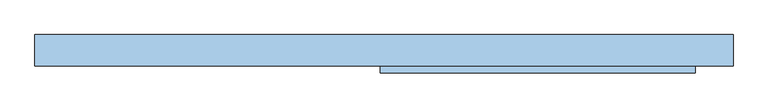
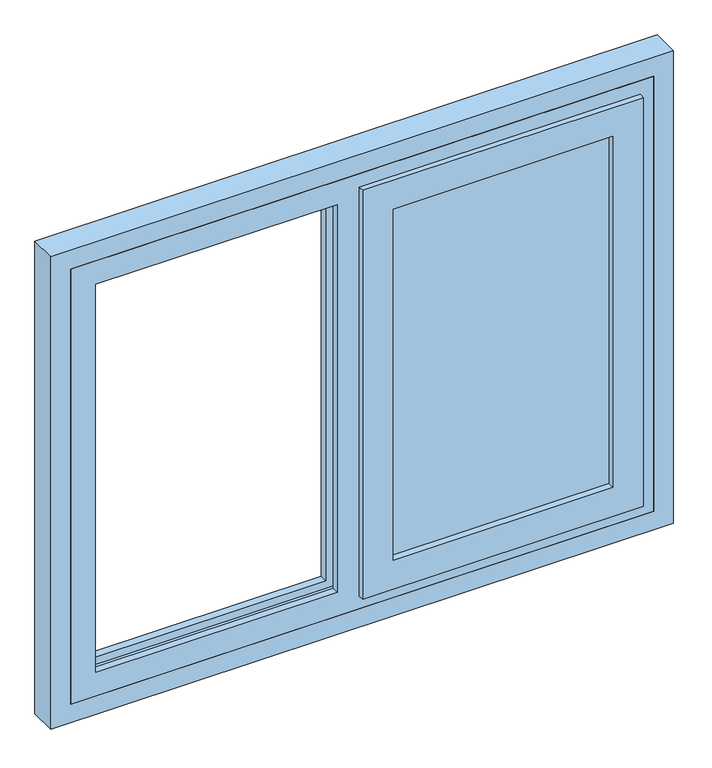
"""IFC4 building model written with IfcOpenShell, lengths in millimetres: window geometry, Окно 2-Откидное - Левое глухое - Один переплет с многокамерным стеклопакетом - 30674-99 : ОП Г1  1160-1540 (4M1-10-4M1-10-4M1) ГОСТ 30674-99."""

from ifc_helpers import new_model, si_unit, frame, origin, place, context, project, spatial, polyline, outline, extrude, faceted_brep, source, transform, mapped, element, save


def window_171b5b07(model_context):
    return source(origin(), model_context, "Body", "SolidModel", [
        extrude(outline(polyline([(942.0, 643.0), (1918.0, 643.0), (1918.0, 49.0), (942.0, 49.0), (942.0, 643.0)]), holes=[polyline([(1903.0, 628.0), (957.0, 628.0), (957.0, 64.0), (1903.0, 64.0), (1903.0, 628.0)])]), frame((0.0, 140.0, 0.0), z_axis=(0.0, 1.0, 0.0), x_axis=(0.0, 0.0, 1.0)), (0.0, 0.0, 1.0), 10.0),
        extrude(outline(polyline([(942.0, 643.0), (1918.0, 643.0), (1918.0, 49.0), (942.0, 49.0), (942.0, 643.0)]), holes=[polyline([(1903.0, 628.0), (957.0, 628.0), (957.0, 64.0), (1903.0, 64.0), (1903.0, 628.0)])]), frame((0.0, 126.0, 0.0), z_axis=(0.0, 1.0, 0.0), x_axis=(0.0, 0.0, 1.0)), (0.0, 0.0, 1.0), 10.0),
        extrude(outline(polyline([(49.0, 140.0), (643.0, 140.0), (643.0, 136.0), (49.0, 136.0), (49.0, 140.0)])), frame((0.0, 0.0, 942.0), z_axis=(0.0, 0.0, 1.0), x_axis=(1.0, 0.0, 0.0)), (0.0, 0.0, 1.0), 976.0),
        extrude(outline(polyline([(49.0, 154.0), (643.0, 154.0), (643.0, 150.0), (49.0, 150.0), (49.0, 154.0)])), frame((0.0, 0.0, 942.0), z_axis=(0.0, 0.0, 1.0), x_axis=(1.0, 0.0, 0.0)), (0.0, 0.0, 1.0), 976.0),
        extrude(outline(polyline([(49.0, 126.0), (643.0, 126.0), (643.0, 122.0), (49.0, 122.0), (49.0, 126.0)])), frame((0.0, 0.0, 942.0), z_axis=(0.0, 0.0, 1.0), x_axis=(1.0, 0.0, 0.0)), (0.0, 0.0, 1.0), 976.0),
        faceted_brep([(-735.0, 120.0, 2010.0), (-735.0, 190.0, 2010.0), (-735.0, 190.0, 850.0), (-735.0, 120.0, 850.0), (735.0, 190.0, 850.0), (735.0, 190.0, 2010.0), (-672.0, 190.0, 1947.0), (-672.0, 190.0, 913.0), (-63.0, 190.0, 913.0), (-63.0, 190.0, 1947.0), (19.0, 190.0, 1947.0), (19.0, 190.0, 913.0), (672.0, 190.0, 913.0), (672.0, 190.0, 1947.0), (735.0, 120.0, 850.0), (735.0, 120.0, 2010.0), (-672.0, 120.0, 913.0), (-672.0, 120.0, 1947.0), (-63.0, 120.0, 1947.0), (-63.0, 120.0, 913.0), (0.0, 120.0, 893.0), (0.0, 120.0, 1967.0), (692.0, 120.0, 1967.0), (692.0, 120.0, 893.0), (-672.0, 138.0, 1947.0), (-672.0, 138.0, 913.0), (-63.0, 138.0, 913.0), (-692.0, 138.0, 893.0), (-692.0, 138.0, 1967.0), (-43.0, 138.0, 1967.0), (-43.0, 138.0, 893.0), (-63.0, 138.0, 1947.0), (-692.0, 170.0, 1967.0), (-692.0, 170.0, 893.0), (-43.0, 170.0, 893.0), (-43.0, 170.0, 1967.0), (-672.0, 170.0, 913.0), (-672.0, 170.0, 1947.0), (-63.0, 170.0, 1947.0), (-63.0, 170.0, 913.0), (0.0, 176.0, 893.0), (0.0, 176.0, 1967.0), (692.0, 176.0, 893.0), (692.0, 176.0, 1967.0), (19.0, 176.0, 913.0), (19.0, 176.0, 1947.0), (672.0, 176.0, 1947.0), (672.0, 176.0, 913.0)], [[[0, 1, 2, 3]], [[4, 2, 1, 5], [6, 7, 8, 9], [10, 11, 12, 13]], [[3, 2, 4, 14]], [[15, 0, 3, 14], [16, 17, 18, 19], [20, 21, 22, 23]], [[24, 17, 16, 25]], [[25, 16, 19, 26]], [[27, 28, 29, 30], [24, 25, 26, 31]], [[32, 28, 27, 33]], [[33, 27, 30, 34]], [[32, 33, 34, 35], [36, 37, 38, 39]], [[6, 37, 36, 7]], [[7, 36, 39, 8]], [[15, 14, 4, 5]], [[26, 19, 18, 31]], [[34, 30, 29, 35]], [[8, 39, 38, 9]], [[40, 41, 21, 20]], [[42, 43, 41, 40], [44, 45, 46, 47]], [[20, 23, 42, 40]], [[11, 10, 45, 44]], [[47, 12, 11, 44]], [[46, 13, 12, 47]], [[43, 42, 23, 22]], [[5, 1, 0, 15]], [[17, 24, 31, 18]], [[28, 32, 35, 29]], [[37, 6, 9, 38]], [[13, 46, 45, 10]], [[41, 43, 22, 21]]]),
        faceted_brep([(69.0, 174.0, 1898.0), (69.0, 154.0, 1898.0), (69.0, 154.0, 962.0), (69.0, 174.0, 962.0), (49.0, 154.0, 942.0), (643.0, 154.0, 942.0), (643.0, 154.0, 1918.0), (49.0, 154.0, 1918.0), (623.0, 154.0, 1898.0), (623.0, 154.0, 962.0), (623.0, 174.0, 962.0), (12.0, 174.0, 1955.0), (680.0, 174.0, 1955.0), (680.0, 174.0, 905.0), (12.0, 174.0, 905.0), (623.0, 174.0, 1898.0), (12.0, 118.0, 1955.0), (12.0, 118.0, 905.0), (680.0, 118.0, 905.0), (-8.0, 118.0, 1975.0), (700.0, 118.0, 1975.0), (700.0, 118.0, 885.0), (-8.0, 118.0, 885.0), (680.0, 118.0, 1955.0), (-8.0, 104.0, 1975.0), (-8.0, 104.0, 885.0), (700.0, 104.0, 885.0), (700.0, 104.0, 1975.0), (69.0, 104.0, 1898.0), (623.0, 104.0, 1898.0), (623.0, 104.0, 962.0), (69.0, 104.0, 962.0), (69.0, 122.0, 1898.0), (69.0, 122.0, 962.0), (623.0, 122.0, 962.0), (49.0, 122.0, 1918.0), (643.0, 122.0, 1918.0), (643.0, 122.0, 942.0), (49.0, 122.0, 942.0), (623.0, 122.0, 1898.0)], [[[0, 1, 2, 3]], [[4, 5, 6, 7], [1, 8, 9, 2]], [[3, 2, 9, 10]], [[11, 12, 13, 14], [3, 10, 15, 0]], [[16, 11, 14, 17]], [[17, 14, 13, 18]], [[19, 20, 21, 22], [17, 18, 23, 16]], [[24, 19, 22, 25]], [[25, 22, 21, 26]], [[25, 26, 27, 24], [28, 29, 30, 31]], [[32, 28, 31, 33]], [[33, 31, 30, 34]], [[35, 36, 37, 38], [33, 34, 39, 32]], [[7, 35, 38, 4]], [[4, 38, 37, 5]], [[10, 9, 8, 15]], [[18, 13, 12, 23]], [[26, 21, 20, 27]], [[34, 30, 29, 39]], [[5, 37, 36, 6]], [[15, 8, 1, 0]], [[23, 12, 11, 16]], [[27, 20, 19, 24]], [[39, 29, 28, 32]], [[6, 36, 35, 7]]]),
        extrude(outline(polyline([(800.0, -785.0), (800.0, 785.0), (2060.0, 785.0), (2060.0, -785.0), (800.0, -785.0)]), holes=[polyline([(2010.0, -735.0), (2010.0, 735.0), (850.0, 735.0), (850.0, -735.0), (2010.0, -735.0)])]), frame((0.0, 120.0, 0.0), z_axis=(0.0, 1.0, 0.0), x_axis=(0.0, 0.0, 1.0)), (0.0, 0.0, 1.0), 70.0),
    ])


if __name__ == "__main__":
    model = new_model("IFC4")
    model_context = context("Model", 3, world=origin())
    ifc_project = project(units=[si_unit("LENGTHUNIT", "METRE", prefix="MILLI")], contexts=[model_context])
    site = spatial("IfcSite", under=ifc_project)
    building = spatial("IfcBuilding", under=site)
    placement = place(None, origin())
    window_shape = window_171b5b07(model_context)
    element("IfcWindow", 1, ObjectType="Окно 2-Откидное - Левое глухое - Один переплет с многокамерным стеклопакетом - 30674-99 : ОП Г1  1160-1540 (4M1-10-4M1-10-4M1) ГОСТ 30674-99", at=placement, inside=building, context=model_context, shape_type="MappedRepresentation", body=[
        mapped(window_shape, transform((0.0, 0.0, 0.0), x_axis=(1.0, 0.0, 0.0), y_axis=(0.0, 1.0, 0.0), z_axis=(0.0, 0.0, 1.0))),
    ])
    save(model, "model.ifc")

# Revit data of these elements
# Type "Окно 2-Откидное - Левое глухое - Один переплет с многокамерным стеклопакетом - 30674-99 : ОП Г1  1160-1540 (4M1-10-4M1-10-4M1) ГОСТ 30674-99"
#   Type Mark = "109"
#   Description = "ОП Г1  1200-1400 (4M1-10-4M1-10-4M1) ГОСТ 30674-99"
#   Вставка окна [instance default] = 0 mm
#   Visual Light Transmittance = 0.9
#   Solar Heat Gain Coefficient = 0.78
#   Ширина переплета 1 = 77 mm
#   Rough Width = 1570 mm
#   Rough Height = 1260 mm
#   Height = 1160 mm
#   Толщина_Тепл_Изоляции = 50 mm
#   Heat Transfer Coefficient (U) = 3.6886 W/(m²·K)
#   G = 32 mm
#   Ширина каркаса = 63 mm
#   Высота подоконника по умолчанию = 800 mm
#   Width = 1470 mm
#   Трехкамерный стеклопакет = yes
#   Двухкамерный стеклопакет = no
#   Переплет = Деревянный переплет
#   Тепловая изоляция = Тепловая изоляция
#   Оконное стекло = Стекло
#   Кадр = Деревянный каркас
#   Construction Type Id = ""
#   Wall Closure = (empty or 0)
#   Analytic Construction = (empty or 0)
# Element 1 (IfcWindow, "Окно 2-Откидное - Левое глухое - Один переплет с многокамерным стеклопакетом - 30674-99 : ОП Г1  1160-1540 (4M1-10-4M1-10-4M1) ГОСТ 30674-99")
#   Materials on its faces: "Деревянный каркас", "Деревянный переплет", "Алюминий", "Стекло", "Тепловая изоляция"
# Materials
#   "Деревянный переплет": class "Древесина", colour RGB 224 176 126, transparency 0, Cost = 0
#   "Тепловая изоляция": class "Пластмасса", colour RGB 185 154 119, transparency 0, Cost = 0
#   "Стекло": class "Стекло", colour RGB 0 0 255, transparency 0.75
#   "Деревянный каркас": class "Древесина", colour RGB 224 176 126, transparency 0, Cost = 0
#   "Алюминий": class "Металл", colour RGB 247 247 247, transparency 0
